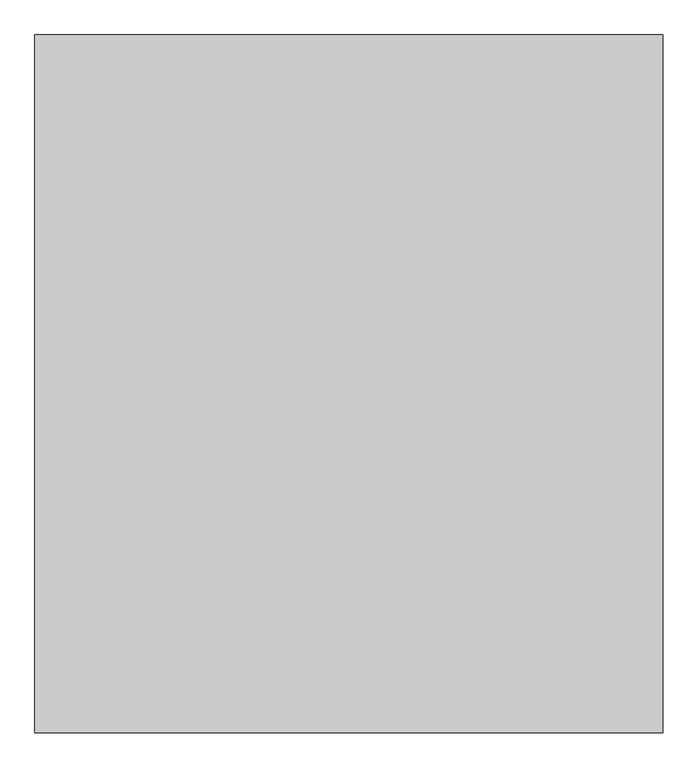
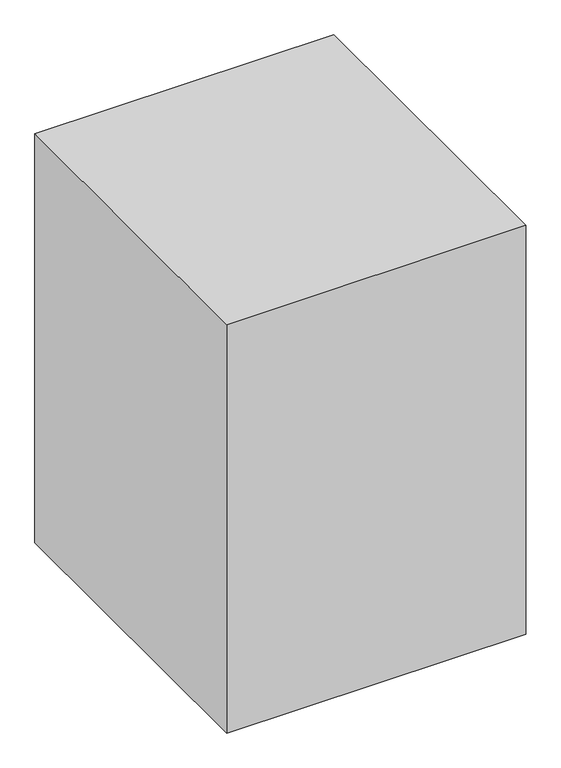
"""IFC4 building model written with IfcOpenShell, lengths in millimetres: proxy geometry, Space Planning Box_hec : Space Planning Box_hec."""

from ifc_helpers import new_model, si_unit, origin, origin_with_axes, place, context, project, spatial, polyline, outline, extrude, source, transform, mapped, element, save


def generic_models_2b76ab57(model_context):
    return source(origin(), model_context, "Body", "SweptSolid", [
        extrude(outline(polyline([(1800.0, 2000.0), (1800.0, -2000.0), (-1800.0, -2000.0), (-1800.0, 2000.0), (1800.0, 2000.0)])), origin_with_axes(), (0.0, 0.0, 1.0), 5200.0),
    ])


if __name__ == "__main__":
    model = new_model("IFC4")
    model_context = context("Model", 3, world=origin())
    ifc_project = project(units=[si_unit("LENGTHUNIT", "METRE", prefix="MILLI")], contexts=[model_context])
    site = spatial("IfcSite", under=ifc_project)
    building = spatial("IfcBuilding", under=site)
    placement = place(None, origin())
    generic_models_shape = generic_models_2b76ab57(model_context)
    element("IfcBuildingElementProxy", 1, Name="Space Planning Box_hec : Space Planning Box_hec", ObjectType="Space Planning Box_hec : Space Planning Box_hec", at=placement, inside=building, context=model_context, shape_type="MappedRepresentation", body=[
        mapped(generic_models_shape, transform((0.0, 0.0, 0.0), x_axis=(1.0, 0.0, 0.0), y_axis=(0.0, 1.0, 0.0), z_axis=(0.0, 0.0, 1.0))),
    ])
    save(model, "model.ifc")

# Revit data of these elements
# Type "Space Planning Box_hec : Space Planning Box_hec"
#   Type Comments = "..."
#   Room Name [instance default] = "?"
#   Interior Finish [instance default] = ""
#   Exterior Finish [instance default] = ""
#   Department [instance default] = ""
#   Assembly Code = "..."
#   ceiling height [instance default] = 0
#   Width [instance default] = 1524 mm
#   Program Area [instance default] = 0.00 m²
#   Length [instance default] = 1524 mm
#   Height [instance default] = 1524 mm
#   Area [instance default] = 2.32258 m²
#   Fill Color [instance default] = Cyan
#   Default Elevation = 0
# Element 1 (IfcBuildingElementProxy, "Space Planning Box_hec : Space Planning Box_hec")
#   Room Name = "Toilet (M)"
#   Interior Finish = "IW3..N/A,,N/A..N/A,,FL5..N/A,,CL5..N/A"
#   Exterior Finish = "N/A..N/A,,EW1..N/A"
#   Department = "AR"
#   ceiling height = 2400
#   Width = 3600 mm
#   Program Area = 14.40 m²
#   Length = 4000 mm
#   Height = 5200 mm
#   Area = 14.40 m²
#   Materials on its faces: "Cyan"
# Materials
#   "Cyan": class "Generic", colour RGB 0 255 255, transparency 0.2, Cost = 0
